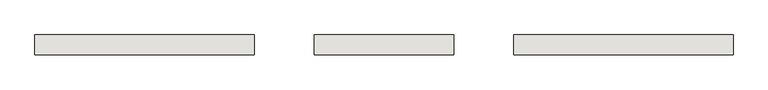
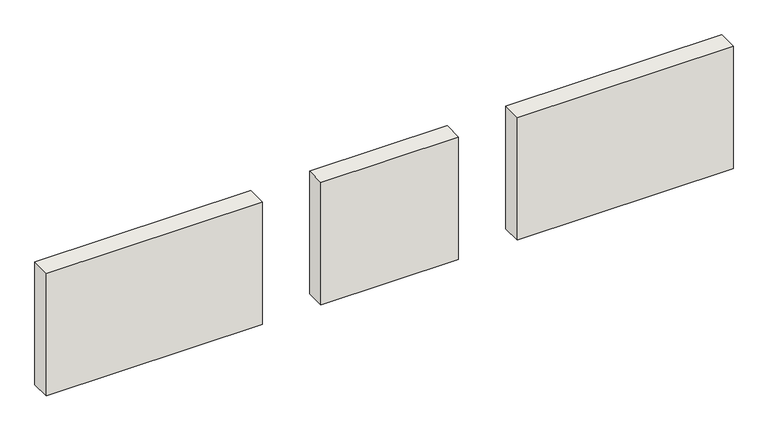
"""IFC4 building model written with IfcOpenShell, lengths in millimetres: wall geometry, 0_3d."""

from ifc_helpers import new_model, si_unit, origin, origin_with_axes, place, context, project, spatial, polyline, outline, extrude, source, transform, mapped, element, save


def wall_88b4bd1f(model_context):
    return source(origin(), model_context, "Body", "SweptSolid", [
        extrude(outline(polyline([(4160.0, 380.0), (4160.0, 0.0), (0.0, 0.0), (0.0, 380.0), (4160.0, 380.0)])), origin_with_axes(), (0.0, 0.0, 1.0), 2500.0),
        extrude(outline(polyline([(5295.0, 0.0), (5295.0, 380.0), (7945.0, 380.0), (7945.0, 0.0), (5295.0, 0.0)])), origin_with_axes(), (0.0, 0.0, 1.0), 2500.0),
        extrude(outline(polyline([(9080.0, 0.0), (9080.0, 380.0), (13240.0, 380.0), (13240.0, 0.0), (9080.0, 0.0)])), origin_with_axes(), (0.0, 0.0, 1.0), 2500.0),
    ])


if __name__ == "__main__":
    model = new_model("IFC4")
    model_context = context("Model", 3, world=origin())
    ifc_project = project(units=[si_unit("LENGTHUNIT", "METRE", prefix="MILLI")], contexts=[model_context])
    site = spatial("IfcSite", under=ifc_project)
    building = spatial("IfcBuilding", under=site)
    placement = place(None, origin())
    wall_shape = wall_88b4bd1f(model_context)
    element("IfcWall", 1, ObjectType="0_3d", at=placement, inside=building, context=model_context, shape_type="MappedRepresentation", body=[
        mapped(wall_shape, transform((0.0, 0.0, 0.0), x_axis=(1.0, 0.0, 0.0), y_axis=(0.0, 1.0, 0.0), z_axis=(0.0, 0.0, 1.0))),
    ])
    save(model, "model.ifc")

# Revit data of these elements
# Element 1 (IfcWall, "0_3d")
#   Materials on its faces: "holzschalung"
# Materials
#   "holzschalung": class "Unassigned", colour RGB 128 128 128, transparency 0
